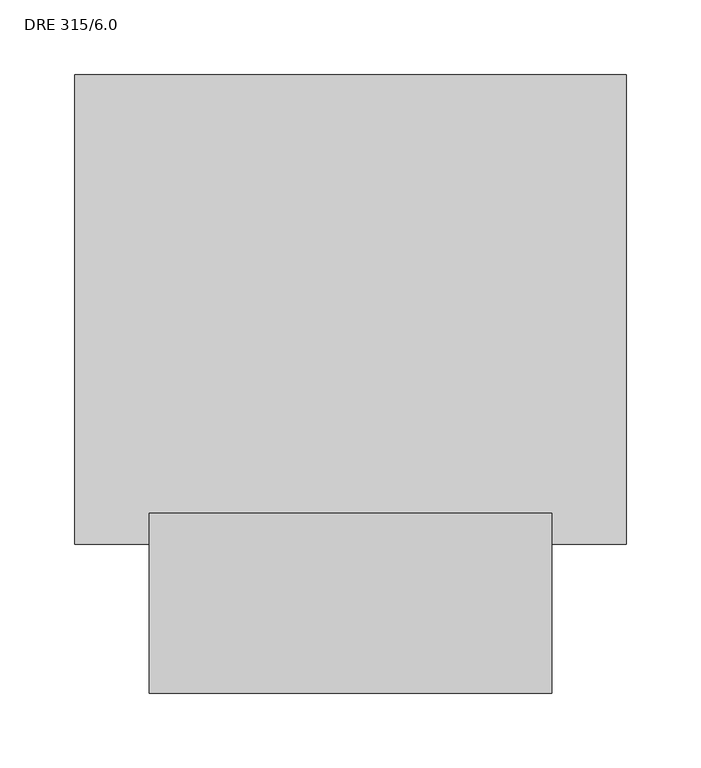
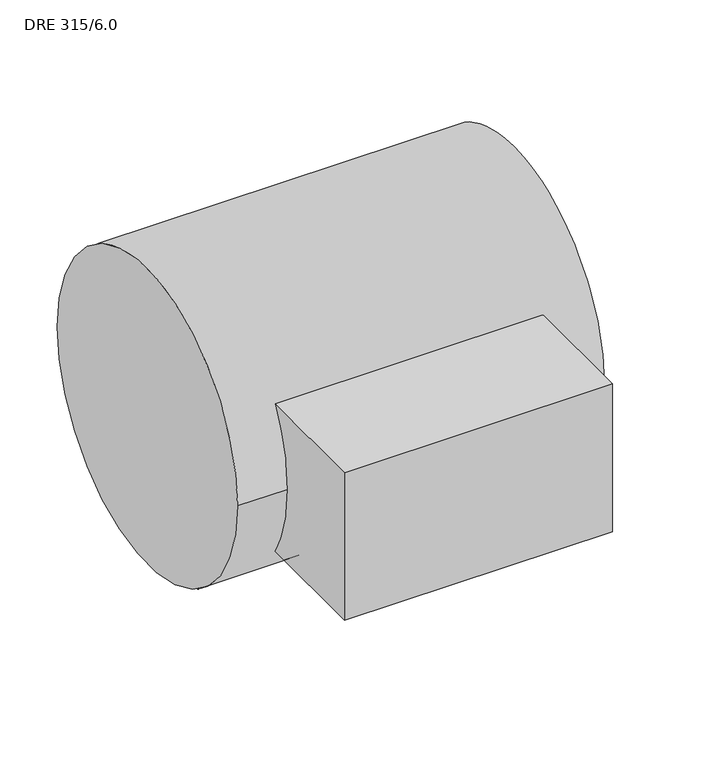
"""IFC4 building model written with IfcOpenShell, lengths in millimetres: proxy geometry, Воздухонагреватель DRE : DRE 315/6.0."""

from ifc_helpers import new_model, si_unit, frame, origin, place, context, project, spatial, circle_curve, source, transform, mapped, element, save
from ifc_brep_helpers import plane_surface, cylinder_surface, advanced_brep


def dre_315_6_0_63bd327c(model_context):
    return source(origin(), model_context, "Body", "AdvancedBrep", [
        advanced_brep(
        [(185.0, -157.5, 0.0), (185.0, 157.5, 0.0), (-185.0, -157.5, 0.0), (-185.0, 157.5, 0.0), (135.0, -157.5, 0.0), (135.0, -136.3990011, -78.75), (-135.0, -136.3990011, -78.75), (-135.0, -157.5, 0.0), (-135.0, -136.3990011, 78.75), (135.0, -136.3990011, 78.75), (135.0, -257.5, 78.75), (135.0, -257.5, -78.75), (-135.0, -257.5, -78.75), (-135.0, -257.5, 78.75)],
        [
            (0, 1, circle_curve(frame((185.0, 0.0, 0.0), z_axis=(1.0, 0.0, 0.0), x_axis=(0.0, 1.0, 0.0)), 157.5)),
            (1, 0, circle_curve(frame((185.0, 0.0, 0.0), z_axis=(1.0, 0.0, 0.0), x_axis=(0.0, 1.0, 0.0)), 157.5)),
            (2, 3, circle_curve(frame((-185.0, 0.0, 0.0), z_axis=(-1.0, 0.0, 0.0), x_axis=(0.0, 1.0, 0.0)), 157.5)),
            (3, 2, circle_curve(frame((-185.0, 0.0, 0.0), z_axis=(-1.0, 0.0, 0.0), x_axis=(0.0, 1.0, 0.0)), 157.5)),
            (0, 4),
            (4, 5, circle_curve(frame((135.0, 0.0, 0.0), z_axis=(1.0, 0.0, 0.0), x_axis=(0.0, 1.0, 0.0)), 157.5)),
            (5, 6),
            (6, 7, circle_curve(frame((-135.0, 0.0, 0.0), z_axis=(-1.0, 0.0, 0.0), x_axis=(0.0, 1.0, 0.0)), 157.5)),
            (7, 2),
            (3, 1),
            (7, 8, circle_curve(frame((-135.0, 0.0, 0.0), z_axis=(-1.0, 0.0, 0.0), x_axis=(0.0, 1.0, 0.0)), 157.5)),
            (8, 9),
            (9, 4, circle_curve(frame((135.0, 0.0, 0.0), z_axis=(1.0, 0.0, 0.0), x_axis=(0.0, 1.0, 0.0)), 157.5)),
            (10, 11),
            (11, 5),
            (9, 10),
            (12, 13),
            (13, 8),
            (6, 12),
            (13, 10),
            (12, 11),
        ],
        [
            plane_surface(frame((185.0, 157.5, 0.0), z_axis=(1.0, 0.0, 0.0), x_axis=(0.0, 0.0, 1.0))),
            plane_surface(frame((-185.0, 157.5, 0.0), z_axis=(-1.0, 0.0, 0.0), x_axis=(0.0, 0.0, -1.0))),
            cylinder_surface(frame((-185.0, 0.0, 0.0), z_axis=(1.0, 0.0, 0.0), x_axis=(0.0, 1.0, 0.0)), 157.5),
            plane_surface(frame((135.0, -257.5, 78.75), z_axis=(1.0, 0.0, 0.0), x_axis=(0.0, -1.0, 0.0))),
            plane_surface(frame((-135.0, -257.5, 78.75), z_axis=(-1.0, 0.0, 0.0), x_axis=(0.0, 1.0, 0.0))),
            plane_surface(frame((135.0, 0.0, 78.75), z_axis=(0.0, 0.0, 1.0), x_axis=(-1.0, 0.0, 0.0))),
            plane_surface(frame((135.0, -257.5, 78.75), z_axis=(0.0, -1.0, 0.0), x_axis=(-1.0, 0.0, 0.0))),
            plane_surface(frame((135.0, -257.5, -78.75), z_axis=(0.0, 0.0, -1.0), x_axis=(-1.0, 0.0, 0.0))),
        ],
        [
            (0, [[1, 2]]),
            (1, [[3, 4]]),
            (2, [[-1, 5, 6, 7, 8, 9, -4, 10]]),
            (2, [[-2, -10, -3, -9, 11, 12, 13, -5]]),
            (3, [[14, 15, -6, -13, 16]]),
            (4, [[17, 18, -11, -8, 19]]),
            (5, [[20, -16, -12, -18]]),
            (6, [[-14, -20, -17, 21]]),
            (7, [[-21, -19, -7, -15]]),
        ],
    ),
    ])


if __name__ == "__main__":
    model = new_model("IFC4")
    model_context = context("Model", 3, world=origin())
    ifc_project = project(units=[si_unit("LENGTHUNIT", "METRE", prefix="MILLI")], contexts=[model_context])
    site = spatial("IfcSite", under=ifc_project)
    building = spatial("IfcBuilding", under=site)
    placement = place(None, origin())
    dre_315_6_0_shape = dre_315_6_0_63bd327c(model_context)
    element("IfcBuildingElementProxy", 1, Name="Воздухонагреватель DRE : DRE 315/6.0", ObjectType="Воздухонагреватель DRE : DRE 315/6.0", at=placement, inside=building, context=model_context, shape_type="MappedRepresentation", body=[
        mapped(dre_315_6_0_shape, transform((0.0, 0.0, 0.0), x_axis=(1.0, 0.0, 0.0), y_axis=(0.0, 1.0, 0.0), z_axis=(0.0, 0.0, 1.0))),
    ])
    save(model, "model.ifc")

# Revit data of these elements
# Type "Воздухонагреватель DRE : DRE 315/6.0"
#   ADSK_Система_Имя [instance default] = ""
#   ADSK_Наименование краткое = "DRE 315/6.0"
#   ADSK_Наименование [instance default] = "Воздухонагреватель DRE 315/6.0"
#   ADSK_Масса_Текст = "8.86"
#   ADSK_Марка = ""
#   ADSK_Код изделия = ""
#   ADSK_Завод-изготовитель = "WAER"
#   ADSK_Единица измерения = "шт."
#   ADSK_URL страницы изделия = ""
#   ADSK_URL документации изделия = ""
#   ширина нагрева = 157.5 mm
#   высота нагрева = 257.5 mm
#   ADSK_Ток = 9.11606 A
#   ADSK_Тепловая мощность = 6000 W
#   ADSK_Расход воздуха = 0 m³/h
#   ADSK_Размер_Длина_L = 370 mm
#   ADSK_Размер_Диаметр_D = 315 mm
#   ADSK_Потеря давления воздуха = 0.0 Pa
#   ADSK_Полная мощность = 6000 VA
#   ADSK_Номинальная мощность = 6000 W
#   ADSK_Напряжение = 380 V
#   ADSK_Масса = 8.86
#   ADSK_Количество ступеней = 1 mm
#   ADSK_Количество [instance default] = 1
#   ADSK_Количество фаз = 3
#   ADSK_Классификация нагрузок = ОВК
#   Default Elevation = 0
#   URL = ""
#   Cost = 0
